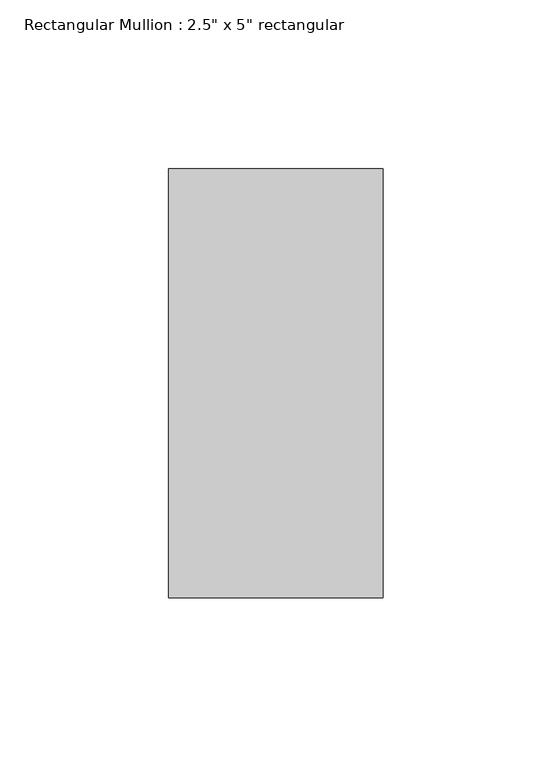
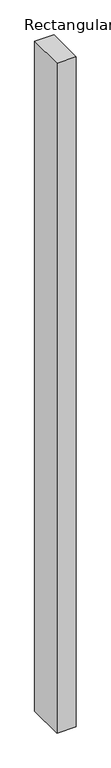
"""IFC4 building model written with IfcOpenShell, lengths in millimetres: member geometry."""

import ifcopenshell
import ifcopenshell.guid

model = None  # the IFC model being written
_history = None  # IfcOwnerHistory: only IFC2X3 demands one
_inside = {}  # id of a spatial element -> (the spatial element, [elements in it])
_under = {}  # id of a project, library or spatial element -> (it, [spatial elements below it])
_declared = {}  # id of a project -> (the project, [libraries it declares])
_typed = {}  # id of a type object -> (the type object, [elements of that type])
_made_of = {}  # id of a material, layer set ... -> (it, [elements and type objects made of it])


def new_model(schema):
    """Start an empty IFC model of exactly this schema.

    Asked for "IFC4X3", IfcOpenShell would pick the latest addendum, in which some entities
    have other attributes; the version numbers below select the first issue.
    IFC2X3 requires an IfcOwnerHistory on every rooted entity: one is made here for all.
    """
    global model, _history
    if schema == "IFC4X3":
        model = ifcopenshell.file(schema_version=(4, 3, 0, 0))
    else:
        model = ifcopenshell.file(schema=schema)
    _inside.clear()
    _under.clear()
    _declared.clear()
    _typed.clear()
    _made_of.clear()
    _history = None
    if model.schema == "IFC2X3":
        org = make("IfcOrganization", Name="unknown")
        user = make(
            "IfcPersonAndOrganization",
            ThePerson=make("IfcPerson", FamilyName="unknown"),
            TheOrganization=org,
        )
        app = make(
            "IfcApplication",
            ApplicationDeveloper=org,
            Version="unknown",
            ApplicationFullName="unknown",
            ApplicationIdentifier="unknown",
        )
        _history = make(
            "IfcOwnerHistory",
            OwningUser=user,
            OwningApplication=app,
            ChangeAction="ADDED",
            CreationDate=0,
        )
    return model


def make(cls, **values):
    """One entity of the class cls with the attributes given. An attribute that is None is left unset."""
    return model.create_entity(
        cls, **{name: value for name, value in values.items() if value is not None}
    )


def rooted(cls, **values):
    """An entity with a GlobalId (a new one), such as an element, a storey or a relation."""
    return make(cls, GlobalId=ifcopenshell.guid.new(), OwnerHistory=_history, **values)


def si_unit(unit_type, name, prefix=None):
    """IfcSIUnit, for example si_unit("LENGTHUNIT", "METRE", prefix="MILLI")."""
    return make("IfcSIUnit", UnitType=unit_type, Prefix=prefix, Name=name)


def assignment(units):
    """IfcUnitAssignment: the units of a project."""
    return None if units is None else make("IfcUnitAssignment", Units=units)


def point(xyz):
    """IfcCartesianPoint."""
    return None if xyz is None else make("IfcCartesianPoint", Coordinates=xyz)


def direction(xyz):
    """IfcDirection."""
    return None if xyz is None else make("IfcDirection", DirectionRatios=xyz)


def frame(location, z_axis=None, x_axis=None):
    """IfcAxis2Placement3D, a coordinate frame: its origin and axes. An axis left out is left unset."""
    return make(
        "IfcAxis2Placement3D",
        Location=point(location),
        Axis=direction(z_axis),
        RefDirection=direction(x_axis),
    )


def origin():
    """The frame at (0, 0, 0) with its axes left unset."""
    return frame((0.0, 0.0, 0.0))


def place(relative_to, where):
    """IfcLocalPlacement: puts the frame where relative to a parent placement (None: the world)."""
    return make(
        "IfcLocalPlacement", PlacementRelTo=relative_to, RelativePlacement=where
    )


def context(
    kind, dimensions, precision=None, world=None, true_north=None, identifier=None
):
    """IfcGeometricRepresentationContext, for example the 3D "Model" context."""
    return make(
        "IfcGeometricRepresentationContext",
        ContextIdentifier=identifier,
        ContextType=kind,
        CoordinateSpaceDimension=dimensions,
        Precision=precision,
        WorldCoordinateSystem=world,
        TrueNorth=true_north,
    )


def project(units=None, contexts=None):
    """IfcProject with its units and contexts."""
    return rooted(
        "IfcProject",
        Name="project",
        RepresentationContexts=contexts,
        UnitsInContext=assignment(units),
    )


def spatial(cls, under=None, at=None, **own):
    """A site, building, storey or space (cls), placed at a placement, below another one or the project."""
    s = rooted(cls, ObjectPlacement=at, **own)
    if under is not None:
        _under.setdefault(under.id(), (under, []))[1].append(s)
    return s


def polyline(points):
    """IfcPolyline through the points."""
    return make("IfcPolyline", Points=[point(p) for p in points])


def outline(outer, holes=None, kind="AREA"):
    """IfcArbitraryClosedProfileDef: a profile drawn as a closed curve; with holes, ...WithVoids."""
    if holes is None:
        return make("IfcArbitraryClosedProfileDef", ProfileType=kind, OuterCurve=outer)
    return make(
        "IfcArbitraryProfileDefWithVoids",
        ProfileType=kind,
        OuterCurve=outer,
        InnerCurves=holes,
    )


def extrude(swept, where, along, depth):
    """IfcExtrudedAreaSolid: the profile swept, set in the frame where, extruded along a direction by depth."""
    return make(
        "IfcExtrudedAreaSolid",
        SweptArea=swept,
        Position=where,
        ExtrudedDirection=direction(along),
        Depth=depth,
    )


def shape(context_of_items, identifier, shape_type, items):
    """IfcShapeRepresentation: the items that make up one representation, for example the "Body"."""
    return make(
        "IfcShapeRepresentation",
        ContextOfItems=context_of_items,
        RepresentationIdentifier=identifier,
        RepresentationType=shape_type,
        Items=items,
    )


def source(mapping_origin, context_of_items, identifier, shape_type, items):
    """IfcRepresentationMap: a shape defined once, which mapped items show again and again."""
    return make(
        "IfcRepresentationMap",
        MappingOrigin=mapping_origin,
        MappedRepresentation=shape(context_of_items, identifier, shape_type, items),
    )


def transform(
    local_origin,
    x_axis=None,
    y_axis=None,
    z_axis=None,
    scale=None,
    scale2=None,
    scale3=None,
    uniform=True,
):
    """IfcCartesianTransformationOperator3D, or its non-uniform kind. x_axis, y_axis, z_axis: its Axis1, 2, 3."""
    if uniform:
        return make(
            "IfcCartesianTransformationOperator3D",
            Axis1=direction(x_axis),
            Axis2=direction(y_axis),
            LocalOrigin=point(local_origin),
            Scale=scale,
            Axis3=direction(z_axis),
        )
    return make(
        "IfcCartesianTransformationOperator3DnonUniform",
        Axis1=direction(x_axis),
        Axis2=direction(y_axis),
        LocalOrigin=point(local_origin),
        Scale=scale,
        Axis3=direction(z_axis),
        Scale2=scale2,
        Scale3=scale3,
    )


def mapped(mapping_source, mapping_target):
    """IfcMappedItem: shows the shape of a source again, moved by a transform."""
    return make(
        "IfcMappedItem", MappingSource=mapping_source, MappingTarget=mapping_target
    )


def made_of(thing, what):
    """Note that an element or type object is made of a material, layer set ...; save() writes the relation."""
    if what is not None:
        _made_of.setdefault(what.id(), (what, []))[1].append(thing)
    return thing


def element(
    cls,
    number,
    at=None,
    inside=None,
    cuts=None,
    type_object=None,
    material=None,
    context=None,
    identifier="Body",
    shape_type=None,
    held_by="IfcProductDefinitionShape",
    body=None,
    shapes=None,
    **own,
):
    """One element of the class cls, such as IfcWall. Its Tag is "e" and its number.

    at: its placement. inside: the storey or other place that contains it. cuts: it is an
    opening in that element (IfcRelVoidsElement). A single representation is given by context,
    identifier, shape_type and body (its items); several are given by shapes. held_by: the class
    of the entity that holds the representations. save() writes the other relations.
    """
    e = rooted(cls, Tag="e%d" % number, ObjectPlacement=at, **own)
    if body is not None:
        shapes = [shape(context, identifier, shape_type, body)]
    if shapes is not None:
        e.Representation = make(held_by, Representations=shapes)
    if inside is not None:
        _inside.setdefault(inside.id(), (inside, []))[1].append(e)
    if cuts is not None:
        rooted(
            "IfcRelVoidsElement", RelatingBuildingElement=cuts, RelatedOpeningElement=e
        )
    if type_object is not None:
        _typed.setdefault(type_object.id(), (type_object, []))[1].append(e)
    return made_of(e, material)


def aggregate(whole, parts):
    """IfcRelAggregates: a whole, such as a stair, and the parts it consists of."""
    return rooted("IfcRelAggregates", RelatingObject=whole, RelatedObjects=parts)


def save(model, path):
    """Write the relations noted so far, then the file.

    IfcRelAggregates (storeys below a building ...), IfcRelContainedInSpatialStructure (elements
    in a storey), IfcRelDefinesByType, IfcRelAssociatesMaterial and IfcRelDeclares: one each for
    every whole, place, type object, material and project.
    """
    for whole, parts in _under.values():
        aggregate(whole, parts)
    for where, things in _inside.values():
        rooted(
            "IfcRelContainedInSpatialStructure",
            RelatedElements=things,
            RelatingStructure=where,
        )
    for kind, things in _typed.values():
        rooted("IfcRelDefinesByType", RelatedObjects=things, RelatingType=kind)
    for what, things in _made_of.values():
        rooted("IfcRelAssociatesMaterial", RelatedObjects=things, RelatingMaterial=what)
    for by, libraries in _declared.values():
        rooted("IfcRelDeclares", RelatingContext=by, RelatedDefinitions=libraries)
    model.write(path)


def member_eadc486f(model_context):
    return source(origin(), model_context, "Body", "SweptSolid", [
        extrude(outline(polyline([(0.0, 63.5), (0.0, -63.5), (-63.5, -63.5), (-63.5, 63.5), (0.0, 63.5)])), frame((0.0, 0.0, -2343.15), z_axis=(0.0, 0.0, 1.0), x_axis=(1.0, 0.0, 0.0)), (0.0, 0.0, 1.0), 2343.15),
    ])


if __name__ == "__main__":
    model = new_model("IFC4")
    model_context = context("Model", 3, world=origin())
    ifc_project = project(units=[si_unit("LENGTHUNIT", "METRE", prefix="MILLI")], contexts=[model_context])
    site = spatial("IfcSite", under=ifc_project)
    building = spatial("IfcBuilding", under=site)
    placement = place(None, origin())
    member_shape = member_eadc486f(model_context)
    element("IfcMember", 1, ObjectType="Rectangular Mullion : 2.5\" x 5\" rectangular", at=placement, inside=building, context=model_context, shape_type="MappedRepresentation", body=[
        mapped(member_shape, transform((0.0, 0.0, 0.0), x_axis=(1.0, 0.0, 0.0), y_axis=(0.0, 1.0, 0.0), z_axis=(0.0, 0.0, 1.0))),
    ])
    save(model, "model.ifc")

# Revit data of these elements
# Type "Rectangular Mullion : 2.5\" x 5\" rectangular"
#   built-in parameter 1007304 = 0.416667 (stored number, unit not read)
#   built-in parameter 1007301 = 0.104167 (stored number, unit not read)
#   built-in parameter 1007300 = 0.104167 (stored number, unit not read)
# Element 1 (IfcMember, "Rectangular Mullion : 2.5\" x 5\" rectangular")
#   Materials on its faces: "Aluminum"
# Materials
#   "Aluminum": class "Metal", colour RGB 247 247 247, transparency 0, Description = "Aluminum 6061", Cost = 0
